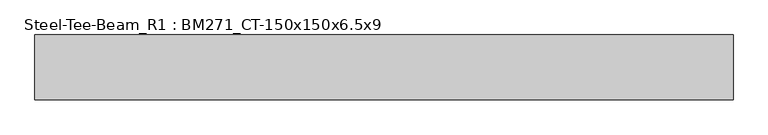
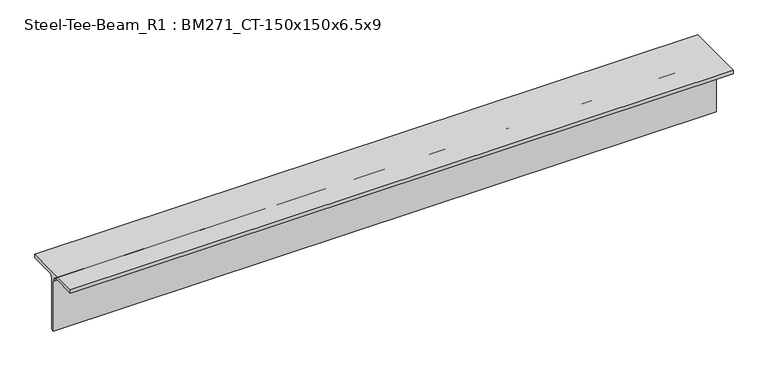
"""IFC4 building model written with IfcOpenShell, lengths in millimetres: member geometry, Steel-Tee-Beam_R1 : BM271_CT-150x150x6.5x9."""

from ifc_helpers import new_model, si_unit, point, frame, frame_2d, origin, place, context, project, spatial, polyline, circle_curve, trimmed, segment, composite_curve, outline, extrude, source, transform, mapped, element, save


def steel_tee_beam_r1_bm271_ct_150x150x6_5x9_a6dc24af(model_context):
    return source(origin(), model_context, "Body", "SweptSolid", [
        extrude(outline(composite_curve([segment(polyline([(-75.0, 75.0), (75.0, 75.0), (75.0, 66.0), (16.25, 66.0)]), True, "CONTINUOUS"), segment(trimmed(circle_curve(frame_2d((16.25, 53.0)), 13.0), [point((16.25, 66.0))], [point((3.25, 53.0))], True, "CARTESIAN"), True, "CONTINUOUS"), segment(polyline([(3.25, 53.0), (3.25, -75.0), (-3.25, -75.0), (-3.25, 53.0)]), True, "CONTINUOUS"), segment(trimmed(circle_curve(frame_2d((-16.25, 53.0)), 13.0), [point((-3.25, 53.0))], [point((-16.25, 66.0))], True, "CARTESIAN"), True, "CONTINUOUS"), segment(polyline([(-16.25, 66.0), (-75.0, 66.0), (-75.0, 75.0)]), True, "CONTINUOUS")], self_intersect=False)), frame((-807.1037633, 0.0, 0.0), z_axis=(1.0, 0.0, 0.0), x_axis=(0.0, 1.0, 0.0)), (0.0, 0.0, 1.0), 1614.2075266),
    ])


if __name__ == "__main__":
    model = new_model("IFC4")
    model_context = context("Model", 3, world=origin())
    ifc_project = project(units=[si_unit("LENGTHUNIT", "METRE", prefix="MILLI")], contexts=[model_context])
    site = spatial("IfcSite", under=ifc_project)
    building = spatial("IfcBuilding", under=site)
    placement = place(None, origin())
    steel_tee_beam_r1_bm271_ct_150x150x6_5x9_shape = steel_tee_beam_r1_bm271_ct_150x150x6_5x9_a6dc24af(model_context)
    element("IfcMember", 1, ObjectType="Steel-Tee-Beam_R1 : BM271_CT-150x150x6.5x9", at=placement, inside=building, context=model_context, shape_type="MappedRepresentation", body=[
        mapped(steel_tee_beam_r1_bm271_ct_150x150x6_5x9_shape, transform((0.0, 0.0, 0.0), x_axis=(1.0, 0.0, 0.0), y_axis=(0.0, 1.0, 0.0), z_axis=(0.0, 0.0, 1.0))),
    ])
    save(model, "model.ifc")

# Revit data of these elements
# Type "Steel-Tee-Beam_R1 : BM271_CT-150x150x6.5x9"
#   Keynote = "CT-150x150x6.5x9"
#   Surface Area = 0.588841 m²/m
#   Section Area = 23.3904 cm²
#   Mass per Unit Length = 18.3614 kg/m
#   Length [instance default] = 1.5240 m
#   bf = 0.1500 m
#   d = 0.1500 m
#   k = 0.0220 m
#   r = 0.0130 m
#   tf = 0.0090 m
#   tw = 0.0065 m
#   hec_material4 [instance default] = none
#   hec_material3 [instance default] = none
#   hec_material2 [instance default] = none
#   hec_material1 [instance default] = none
#   Structural Material [instance default] = Steel, 45-345
#   Assembly Code = ""
# Element 1 (IfcMember, "Steel-Tee-Beam_R1 : BM271_CT-150x150x6.5x9")
#   Structural Material = none
# Materials
#   "Steel, 45-345": class "Metal", colour RGB 189 187 185, transparency 0, Description = "Steel 345 MPa", Cost = 0
